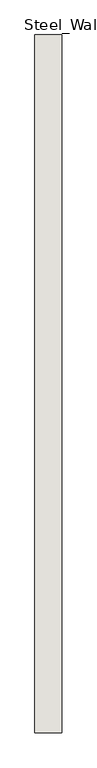
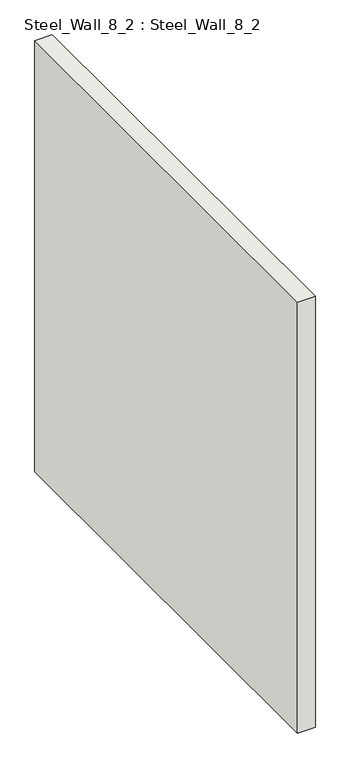
"""IFC4 building model written with IfcOpenShell, lengths in millimetres: wall geometry, Steel_Wall_8_2 : Steel_Wall_8_2."""

from ifc_helpers import new_model, si_unit, frame, origin, place, context, project, spatial, polyline, outline, extrude, source, transform, mapped, element, save


def steel_wall_8_2_steel_wall_8_2_e95248a5(model_context):
    return source(origin(), model_context, "Body", "SweptSolid", [
        extrude(outline(polyline([(6175.0, 14705.0), (6175.0, 12105.0), (6075.0, 12105.0), (6075.0, 14705.0), (6175.0, 14705.0)])), frame((0.0, 0.0, 250.0), z_axis=(0.0, 0.0, 1.0), x_axis=(1.0, 0.0, 0.0)), (0.0, 0.0, 1.0), 2600.0),
    ])


if __name__ == "__main__":
    model = new_model("IFC4")
    model_context = context("Model", 3, world=origin())
    ifc_project = project(units=[si_unit("LENGTHUNIT", "METRE", prefix="MILLI")], contexts=[model_context])
    site = spatial("IfcSite", under=ifc_project)
    building = spatial("IfcBuilding", under=site)
    placement = place(None, origin())
    steel_wall_8_2_steel_wall_8_2_shape = steel_wall_8_2_steel_wall_8_2_e95248a5(model_context)
    element("IfcWall", 1, ObjectType="Steel_Wall_8_2 : Steel_Wall_8_2", at=placement, inside=building, context=model_context, shape_type="MappedRepresentation", body=[
        mapped(steel_wall_8_2_steel_wall_8_2_shape, transform((0.0, 0.0, 0.0), x_axis=(1.0, 0.0, 0.0), y_axis=(0.0, 1.0, 0.0), z_axis=(0.0, 0.0, 1.0))),
    ])
    save(model, "model.ifc")

# Revit data of these elements
# Type "Steel_Wall_8_2 : Steel_Wall_8_2"
#   NameOverride = "Steel_Wall_8_2"
# Element 1 (IfcWall, "Steel_Wall_8_2 : Steel_Wall_8_2")
#   Materials on its faces: "IfcSurfaceStyle #33"
# Materials
#   "IfcSurfaceStyle #33": class "Unassigned", colour RGB 214 214 214, transparency 0
